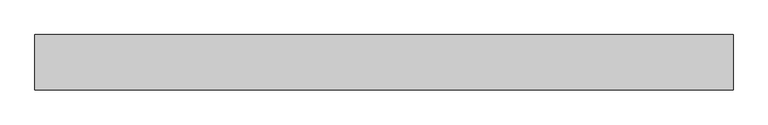
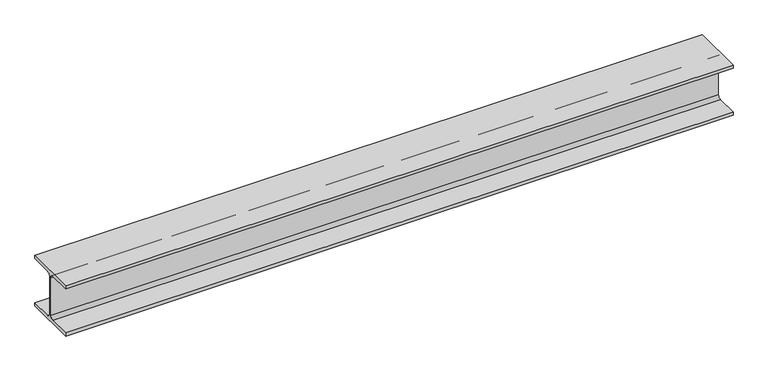
"""IFC4 building model written with IfcOpenShell, lengths in millimetres: beam geometry, 0912_Steel Framing_H-KSD3502 : H_SB_ASB_H-200x200x8x12."""

from ifc_helpers import new_model, si_unit, point, frame, frame_2d, origin, place, context, project, spatial, polyline, circle_curve, trimmed, segment, composite_curve, outline, extrude, source, transform, mapped, element, save


def beam_40c695e5(model_context):
    return source(origin(), model_context, "Body", "SweptSolid", [
        extrude(outline(composite_curve([segment(polyline([(100.0, -88.0), (100.0, -100.0), (-100.0, -100.0), (-100.0, -88.0), (-17.0, -88.0)]), True, "CONTINUOUS"), segment(trimmed(circle_curve(frame_2d((-17.0, -75.0)), 13.0), [point((-17.0, -88.0))], [point((-4.0, -75.0))], True, "CARTESIAN"), True, "CONTINUOUS"), segment(polyline([(-4.0, -75.0), (-4.0, 75.0)]), True, "CONTINUOUS"), segment(trimmed(circle_curve(frame_2d((-17.0, 75.0)), 13.0), [point((-4.0, 75.0))], [point((-17.0, 88.0))], True, "CARTESIAN"), True, "CONTINUOUS"), segment(polyline([(-17.0, 88.0), (-100.0, 88.0), (-100.0, 100.0), (100.0, 100.0), (100.0, 88.0), (17.0, 88.0)]), True, "CONTINUOUS"), segment(trimmed(circle_curve(frame_2d((17.0, 75.0)), 13.0), [point((17.0, 88.0))], [point((4.0, 75.0))], True, "CARTESIAN"), True, "CONTINUOUS"), segment(polyline([(4.0, 75.0), (4.0, -75.0)]), True, "CONTINUOUS"), segment(trimmed(circle_curve(frame_2d((17.0, -75.0)), 13.0), [point((4.0, -75.0))], [point((17.0, -88.0))], True, "CARTESIAN"), True, "CONTINUOUS"), segment(polyline([(17.0, -88.0), (100.0, -88.0)]), True, "CONTINUOUS")], self_intersect=False)), frame((-1256.3461486, 0.0, 0.0), z_axis=(1.0, 0.0, 0.0), x_axis=(0.0, 1.0, 0.0)), (0.0, 0.0, 1.0), 2519.4170066),
    ])


if __name__ == "__main__":
    model = new_model("IFC4")
    model_context = context("Model", 3, world=origin())
    ifc_project = project(units=[si_unit("LENGTHUNIT", "METRE", prefix="MILLI")], contexts=[model_context])
    site = spatial("IfcSite", under=ifc_project)
    building = spatial("IfcBuilding", under=site)
    placement = place(None, origin())
    beam_shape = beam_40c695e5(model_context)
    element("IfcBeam", 1, ObjectType="0912_Steel Framing_H-KSD3502 : H_SB_ASB_H-200x200x8x12", at=placement, inside=building, context=model_context, shape_type="MappedRepresentation", body=[
        mapped(beam_shape, transform((0.0, 0.0, 0.0), x_axis=(1.0, 0.0, 0.0), y_axis=(0.0, 1.0, 0.0), z_axis=(0.0, 0.0, 1.0))),
    ])
    save(model, "model.ifc")

# Revit data of these elements
# Type "0912_Steel Framing_H-KSD3502 : H_SB_ASB_H-200x200x8x12"
#   H_WM Code_1 = "S01AA002-00001 | Main Steel Structure Fabrication Work | Shelter/Building | Medium Steel - Standard (90KG/M>Weight≥30KG/M) | Material: (   )"
#   H_WM Code_2 = "S03AA028-00001 | Main Steel Structure Erection Work | Shelter/Building | Medium Steel (90KG/M>Weight≥30KG/M) | Material: (   )"
#   H_WM Code_3 = "S01AA010-00001 | Main Steel Structure Fabrication Work | Shelter/Building | Steel Painting/Coating | for Non-Fireproofed Steel Surface, Surface Preparation, Primer, Second & Final Coat | Material: (   )"
#   H_Q'ty Cal Type Tag = "SB-Q2"
#   Width = 20.0 cm
#   Web Thickness = 0.8 cm
#   Web Fillet = 1.3 cm
#   Warping Constant = 141000.0 cm⁶
#   W = 0
#   Torsional Moment of Inertia = 26.2485 cm⁴
#   Section Area = 63.53 cm²
#   Plastic Modulus weak axis = 244.0 cm³
#   Plastic Modulus strong axis = 525.0 cm³
#   Perimeter = 1.16 m²/m
#   Nominal Weight = 49.90 kgf/m
#   Moment of Inertia weak axis = 1600.00 cm⁴
#   Moment of Inertia strong axis = 4720.00 cm⁴
#   Height = 20.0 cm
#   Flange Thickness = 1.2 cm
#   Elastic Modulus weak axis = 160.0 cm³
#   Elastic Modulus strong axis = 472.0 cm³
#   Centroid Vertical = 10.0 cm
#   Centroid Horizontal = 10.0 cm
#   Ix = 47200000
#   Length [instance default] = 1.5240 m
#   Zx = 525000
#   b = 0.2000 m
#   h = 0.2000 m
#   r = 0.0130 m
#   s = 0.0080 m
#   t = 0.0120 m
#   A = 0.006353 m²
#   Structural Material [instance default] = Steel, 45-345
#   Assembly Code = ""
# Element 1 (IfcBeam, "0912_Steel Framing_H-KSD3502 : H_SB_ASB_H-200x200x8x12")
#   Structural Material = none
# Materials
#   "Steel, 45-345": class "Metal", colour RGB 189 187 185, transparency 0, Description = "Steel 345 MPa", Cost = 0
